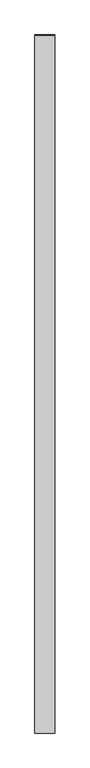
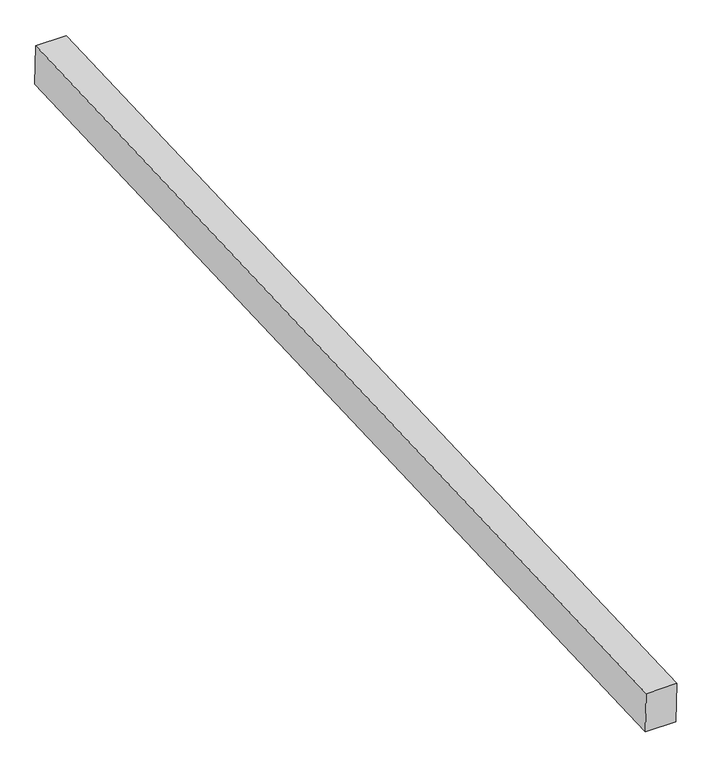
"""IFC4 building model written with IfcOpenShell, lengths in millimetres: proxy geometry, Generic Models 7:Generic Models 1:8:Generic Models 1:8 : Generic Models 7:Generic Models 1:337419:46 : Generic Models 7:Generic Models 1:8:Generic Models 1:8 : Generic Models 7:Generic Models 1:337419:315935."""

import ifcopenshell
import ifcopenshell.guid

model = None  # the IFC model being written
_history = None  # IfcOwnerHistory: only IFC2X3 demands one
_inside = {}  # id of a spatial element -> (the spatial element, [elements in it])
_under = {}  # id of a project, library or spatial element -> (it, [spatial elements below it])
_declared = {}  # id of a project -> (the project, [libraries it declares])
_typed = {}  # id of a type object -> (the type object, [elements of that type])
_made_of = {}  # id of a material, layer set ... -> (it, [elements and type objects made of it])


def new_model(schema):
    """Start an empty IFC model of exactly this schema.

    Asked for "IFC4X3", IfcOpenShell would pick the latest addendum, in which some entities
    have other attributes; the version numbers below select the first issue.
    IFC2X3 requires an IfcOwnerHistory on every rooted entity: one is made here for all.
    """
    global model, _history
    if schema == "IFC4X3":
        model = ifcopenshell.file(schema_version=(4, 3, 0, 0))
    else:
        model = ifcopenshell.file(schema=schema)
    _inside.clear()
    _under.clear()
    _declared.clear()
    _typed.clear()
    _made_of.clear()
    _history = None
    if model.schema == "IFC2X3":
        org = make("IfcOrganization", Name="unknown")
        user = make(
            "IfcPersonAndOrganization",
            ThePerson=make("IfcPerson", FamilyName="unknown"),
            TheOrganization=org,
        )
        app = make(
            "IfcApplication",
            ApplicationDeveloper=org,
            Version="unknown",
            ApplicationFullName="unknown",
            ApplicationIdentifier="unknown",
        )
        _history = make(
            "IfcOwnerHistory",
            OwningUser=user,
            OwningApplication=app,
            ChangeAction="ADDED",
            CreationDate=0,
        )
    return model


def make(cls, **values):
    """One entity of the class cls with the attributes given. An attribute that is None is left unset."""
    return model.create_entity(
        cls, **{name: value for name, value in values.items() if value is not None}
    )


def rooted(cls, **values):
    """An entity with a GlobalId (a new one), such as an element, a storey or a relation."""
    return make(cls, GlobalId=ifcopenshell.guid.new(), OwnerHistory=_history, **values)


def si_unit(unit_type, name, prefix=None):
    """IfcSIUnit, for example si_unit("LENGTHUNIT", "METRE", prefix="MILLI")."""
    return make("IfcSIUnit", UnitType=unit_type, Prefix=prefix, Name=name)


def assignment(units):
    """IfcUnitAssignment: the units of a project."""
    return None if units is None else make("IfcUnitAssignment", Units=units)


def point(xyz):
    """IfcCartesianPoint."""
    return None if xyz is None else make("IfcCartesianPoint", Coordinates=xyz)


def direction(xyz):
    """IfcDirection."""
    return None if xyz is None else make("IfcDirection", DirectionRatios=xyz)


def frame(location, z_axis=None, x_axis=None):
    """IfcAxis2Placement3D, a coordinate frame: its origin and axes. An axis left out is left unset."""
    return make(
        "IfcAxis2Placement3D",
        Location=point(location),
        Axis=direction(z_axis),
        RefDirection=direction(x_axis),
    )


def origin():
    """The frame at (0, 0, 0) with its axes left unset."""
    return frame((0.0, 0.0, 0.0))


def place(relative_to, where):
    """IfcLocalPlacement: puts the frame where relative to a parent placement (None: the world)."""
    return make(
        "IfcLocalPlacement", PlacementRelTo=relative_to, RelativePlacement=where
    )


def context(
    kind, dimensions, precision=None, world=None, true_north=None, identifier=None
):
    """IfcGeometricRepresentationContext, for example the 3D "Model" context."""
    return make(
        "IfcGeometricRepresentationContext",
        ContextIdentifier=identifier,
        ContextType=kind,
        CoordinateSpaceDimension=dimensions,
        Precision=precision,
        WorldCoordinateSystem=world,
        TrueNorth=true_north,
    )


def project(units=None, contexts=None):
    """IfcProject with its units and contexts."""
    return rooted(
        "IfcProject",
        Name="project",
        RepresentationContexts=contexts,
        UnitsInContext=assignment(units),
    )


def spatial(cls, under=None, at=None, **own):
    """A site, building, storey or space (cls), placed at a placement, below another one or the project."""
    s = rooted(cls, ObjectPlacement=at, **own)
    if under is not None:
        _under.setdefault(under.id(), (under, []))[1].append(s)
    return s


def polyline(points):
    """IfcPolyline through the points."""
    return make("IfcPolyline", Points=[point(p) for p in points])


def outline(outer, holes=None, kind="AREA"):
    """IfcArbitraryClosedProfileDef: a profile drawn as a closed curve; with holes, ...WithVoids."""
    if holes is None:
        return make("IfcArbitraryClosedProfileDef", ProfileType=kind, OuterCurve=outer)
    return make(
        "IfcArbitraryProfileDefWithVoids",
        ProfileType=kind,
        OuterCurve=outer,
        InnerCurves=holes,
    )


def extrude(swept, where, along, depth):
    """IfcExtrudedAreaSolid: the profile swept, set in the frame where, extruded along a direction by depth."""
    return make(
        "IfcExtrudedAreaSolid",
        SweptArea=swept,
        Position=where,
        ExtrudedDirection=direction(along),
        Depth=depth,
    )


def shape(context_of_items, identifier, shape_type, items):
    """IfcShapeRepresentation: the items that make up one representation, for example the "Body"."""
    return make(
        "IfcShapeRepresentation",
        ContextOfItems=context_of_items,
        RepresentationIdentifier=identifier,
        RepresentationType=shape_type,
        Items=items,
    )


def source(mapping_origin, context_of_items, identifier, shape_type, items):
    """IfcRepresentationMap: a shape defined once, which mapped items show again and again."""
    return make(
        "IfcRepresentationMap",
        MappingOrigin=mapping_origin,
        MappedRepresentation=shape(context_of_items, identifier, shape_type, items),
    )


def transform(
    local_origin,
    x_axis=None,
    y_axis=None,
    z_axis=None,
    scale=None,
    scale2=None,
    scale3=None,
    uniform=True,
):
    """IfcCartesianTransformationOperator3D, or its non-uniform kind. x_axis, y_axis, z_axis: its Axis1, 2, 3."""
    if uniform:
        return make(
            "IfcCartesianTransformationOperator3D",
            Axis1=direction(x_axis),
            Axis2=direction(y_axis),
            LocalOrigin=point(local_origin),
            Scale=scale,
            Axis3=direction(z_axis),
        )
    return make(
        "IfcCartesianTransformationOperator3DnonUniform",
        Axis1=direction(x_axis),
        Axis2=direction(y_axis),
        LocalOrigin=point(local_origin),
        Scale=scale,
        Axis3=direction(z_axis),
        Scale2=scale2,
        Scale3=scale3,
    )


def mapped(mapping_source, mapping_target):
    """IfcMappedItem: shows the shape of a source again, moved by a transform."""
    return make(
        "IfcMappedItem", MappingSource=mapping_source, MappingTarget=mapping_target
    )


def made_of(thing, what):
    """Note that an element or type object is made of a material, layer set ...; save() writes the relation."""
    if what is not None:
        _made_of.setdefault(what.id(), (what, []))[1].append(thing)
    return thing


def element(
    cls,
    number,
    at=None,
    inside=None,
    cuts=None,
    type_object=None,
    material=None,
    context=None,
    identifier="Body",
    shape_type=None,
    held_by="IfcProductDefinitionShape",
    body=None,
    shapes=None,
    **own,
):
    """One element of the class cls, such as IfcWall. Its Tag is "e" and its number.

    at: its placement. inside: the storey or other place that contains it. cuts: it is an
    opening in that element (IfcRelVoidsElement). A single representation is given by context,
    identifier, shape_type and body (its items); several are given by shapes. held_by: the class
    of the entity that holds the representations. save() writes the other relations.
    """
    e = rooted(cls, Tag="e%d" % number, ObjectPlacement=at, **own)
    if body is not None:
        shapes = [shape(context, identifier, shape_type, body)]
    if shapes is not None:
        e.Representation = make(held_by, Representations=shapes)
    if inside is not None:
        _inside.setdefault(inside.id(), (inside, []))[1].append(e)
    if cuts is not None:
        rooted(
            "IfcRelVoidsElement", RelatingBuildingElement=cuts, RelatedOpeningElement=e
        )
    if type_object is not None:
        _typed.setdefault(type_object.id(), (type_object, []))[1].append(e)
    return made_of(e, material)


def aggregate(whole, parts):
    """IfcRelAggregates: a whole, such as a stair, and the parts it consists of."""
    return rooted("IfcRelAggregates", RelatingObject=whole, RelatedObjects=parts)


def save(model, path):
    """Write the relations noted so far, then the file.

    IfcRelAggregates (storeys below a building ...), IfcRelContainedInSpatialStructure (elements
    in a storey), IfcRelDefinesByType, IfcRelAssociatesMaterial and IfcRelDeclares: one each for
    every whole, place, type object, material and project.
    """
    for whole, parts in _under.values():
        aggregate(whole, parts)
    for where, things in _inside.values():
        rooted(
            "IfcRelContainedInSpatialStructure",
            RelatedElements=things,
            RelatingStructure=where,
        )
    for kind, things in _typed.values():
        rooted("IfcRelDefinesByType", RelatedObjects=things, RelatingType=kind)
    for what, things in _made_of.values():
        rooted("IfcRelAssociatesMaterial", RelatedObjects=things, RelatingMaterial=what)
    for by, libraries in _declared.values():
        rooted("IfcRelDeclares", RelatingContext=by, RelatedDefinitions=libraries)
    model.write(path)


def generic_models_52bc5322(model_context):
    return source(origin(), model_context, "Body", "SweptSolid", [
        extrude(outline(polyline([(-581229.2495411, 3818.908703), (-576356.3266468, 4021.9471569), (-576348.7597251, 3831.5971524), (-581221.3189223, 3628.5738526), (-581229.2495411, 3818.908703)])), frame((614499.411724, 0.0, 0.0), z_axis=(1.0, 0.0, 0.0), x_axis=(0.0, 1.0, 0.0)), (0.0, 0.0, 1.0), 139.7),
    ])


if __name__ == "__main__":
    model = new_model("IFC4")
    model_context = context("Model", 3, world=origin())
    ifc_project = project(units=[si_unit("LENGTHUNIT", "METRE", prefix="MILLI")], contexts=[model_context])
    site = spatial("IfcSite", under=ifc_project)
    building = spatial("IfcBuilding", under=site)
    placement = place(None, origin())
    generic_models_shape = generic_models_52bc5322(model_context)
    element("IfcBuildingElementProxy", 1, Name="Generic Models 7:Generic Models 1:8:Generic Models 1:8 : Generic Models 7:Generic Models 1:337419:46 : Generic Models 7:Generic Models 1:8:Generic Models 1:8 : Generic Models 7:Generic Models 1:337419:315935", ObjectType="Generic Models 7:Generic Models 1:8:Generic Models 1:8 : Generic Models 7:Generic Models 1:337419:46 : Generic Models 7:Generic Models 1:8:Generic Models 1:8 : Generic Models 7:Generic Models 1:337419:315935", at=placement, inside=building, context=model_context, shape_type="MappedRepresentation", body=[
        mapped(generic_models_shape, transform((0.0, 0.0, 0.0), x_axis=(1.0, 0.0, 0.0), y_axis=(0.0, 1.0, 0.0), z_axis=(0.0, 0.0, 1.0))),
    ])
    save(model, "model.ifc")

# Revit data of these elements
# Type "Generic Models 7:Generic Models 1:8:Generic Models 1:8 : Generic Models 7:Generic Models 1:337419:46 : Generic Models 7:Generic Models 1:8:Generic Models 1:8 : Generic Models 7:Generic Models 1:337419:315935"
#   NameOverride = "Generic Models 7:Generic Models 1:8:Generic Models 1:8 : Generic Models 7:Generic Models 1:337419:315935"
#   ObjectTypeOverride = "Generic Models 1:8 : Generic Models 7:Generic Models 1:337419"
#   Reference = "Generic Models 1"
#   Tag = "315935"
# Element 1 (IfcBuildingElementProxy, "Generic Models 7:Generic Models 1:8:Generic Models 1:8 : Generic Models 7:Generic Models 1:337419:46 : Generic Models 7:Generic Models 1:8:Generic Models 1:8 : Generic Models 7:Generic Models 1:337419:315935")
#   Materials on its faces: "5 1/2\" X 7 1/2\" EXTERIOR GRADE GLULAM BEAMS"
# Materials
#   "5 1/2\" X 7 1/2\" EXTERIOR GRADE GLULAM BEAMS": class "Wood", colour RGB 183 134 68, transparency 0, Keynote = "M06181300.01", Description = "Pinus Echinata", Cost = 0
